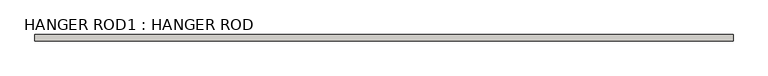
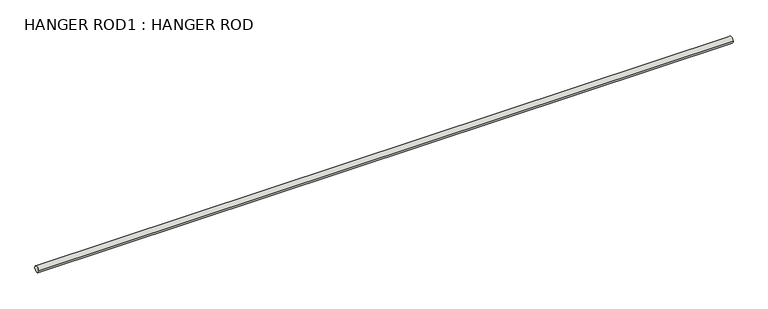
"""IFC4 building model written with IfcOpenShell, lengths in millimetres: wall geometry, HANGER ROD1 : HANGER ROD."""

from ifc_helpers import new_model, si_unit, point, frame, frame_2d, origin, place, context, project, spatial, circle_curve, trimmed, segment, composite_curve, outline, extrude, source, transform, mapped, element, save


def hanger_rod1_hanger_rod_e6e4e40c(model_context):
    return source(origin(), model_context, "Body", "SweptSolid", [
        extrude(outline(composite_curve([segment(trimmed(circle_curve(frame_2d((-1046.4884634, 4908.7706466)), 6.35), [point((-1040.1384634, 4908.7706466))], [point((-1052.8384634, 4908.7706466))], False, "CARTESIAN"), True, "CONTINUOUS"), segment(trimmed(circle_curve(frame_2d((-1046.4884634, 4908.7706466)), 6.35), [point((-1052.8384634, 4908.7706466))], [point((-1040.1384634, 4908.7706466))], False, "CARTESIAN"), True, "CONTINUOUS")], self_intersect=False)), frame((20028.4356381, 0.0, 0.0), z_axis=(1.0, 0.0, 0.0), x_axis=(0.0, 1.0, 0.0)), (0.0, 0.0, 1.0), 1405.2437091),
    ])


if __name__ == "__main__":
    model = new_model("IFC4")
    model_context = context("Model", 3, world=origin())
    ifc_project = project(units=[si_unit("LENGTHUNIT", "METRE", prefix="MILLI")], contexts=[model_context])
    site = spatial("IfcSite", under=ifc_project)
    building = spatial("IfcBuilding", under=site)
    placement = place(None, origin())
    hanger_rod1_hanger_rod_shape = hanger_rod1_hanger_rod_e6e4e40c(model_context)
    element("IfcWall", 1, ObjectType="HANGER ROD1 : HANGER ROD", at=placement, inside=building, context=model_context, shape_type="MappedRepresentation", body=[
        mapped(hanger_rod1_hanger_rod_shape, transform((0.0, 0.0, 0.0), x_axis=(1.0, 0.0, 0.0), y_axis=(0.0, 1.0, 0.0), z_axis=(0.0, 0.0, 1.0))),
    ])
    save(model, "model.ifc")

# Revit data of these elements
# Element 1 (IfcWall, "HANGER ROD1 : HANGER ROD")
#   Materials on its faces: "1/2\" STEEL ROD (RAW STEEL)"
# Materials
#   "1/2\" STEEL ROD (RAW STEEL)": class "Metal", colour RGB 189 187 185, transparency 0, Description = "Structural steel 50ksi", Cost = 0
